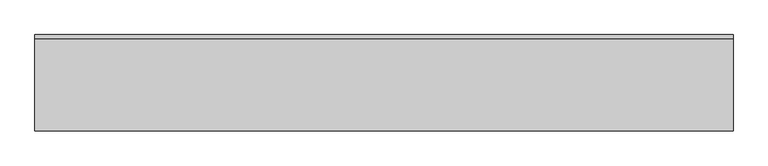
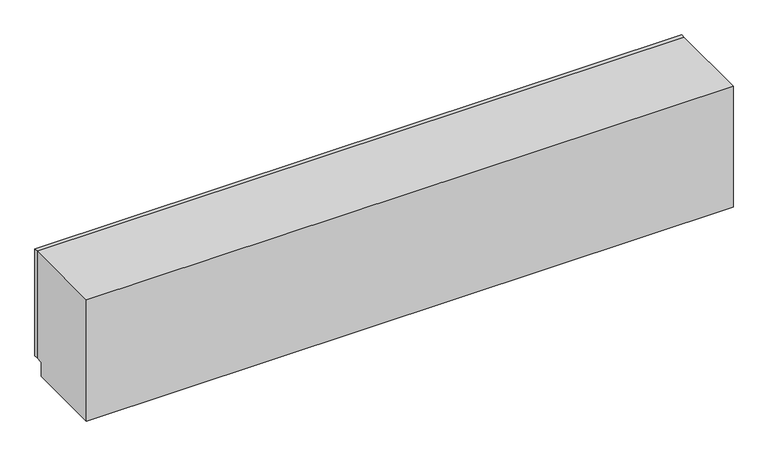
"""IFC4 building model written with IfcOpenShell, lengths in millimetres: furniture geometry, OD_CW_Base Cabinet : OD_CW_Base Cabinet."""

import ifcopenshell
import ifcopenshell.guid

model = None  # the IFC model being written
_history = None  # IfcOwnerHistory: only IFC2X3 demands one
_inside = {}  # id of a spatial element -> (the spatial element, [elements in it])
_under = {}  # id of a project, library or spatial element -> (it, [spatial elements below it])
_declared = {}  # id of a project -> (the project, [libraries it declares])
_typed = {}  # id of a type object -> (the type object, [elements of that type])
_made_of = {}  # id of a material, layer set ... -> (it, [elements and type objects made of it])


def new_model(schema):
    """Start an empty IFC model of exactly this schema.

    Asked for "IFC4X3", IfcOpenShell would pick the latest addendum, in which some entities
    have other attributes; the version numbers below select the first issue.
    IFC2X3 requires an IfcOwnerHistory on every rooted entity: one is made here for all.
    """
    global model, _history
    if schema == "IFC4X3":
        model = ifcopenshell.file(schema_version=(4, 3, 0, 0))
    else:
        model = ifcopenshell.file(schema=schema)
    _inside.clear()
    _under.clear()
    _declared.clear()
    _typed.clear()
    _made_of.clear()
    _history = None
    if model.schema == "IFC2X3":
        org = make("IfcOrganization", Name="unknown")
        user = make(
            "IfcPersonAndOrganization",
            ThePerson=make("IfcPerson", FamilyName="unknown"),
            TheOrganization=org,
        )
        app = make(
            "IfcApplication",
            ApplicationDeveloper=org,
            Version="unknown",
            ApplicationFullName="unknown",
            ApplicationIdentifier="unknown",
        )
        _history = make(
            "IfcOwnerHistory",
            OwningUser=user,
            OwningApplication=app,
            ChangeAction="ADDED",
            CreationDate=0,
        )
    return model


def make(cls, **values):
    """One entity of the class cls with the attributes given. An attribute that is None is left unset."""
    return model.create_entity(
        cls, **{name: value for name, value in values.items() if value is not None}
    )


def rooted(cls, **values):
    """An entity with a GlobalId (a new one), such as an element, a storey or a relation."""
    return make(cls, GlobalId=ifcopenshell.guid.new(), OwnerHistory=_history, **values)


def si_unit(unit_type, name, prefix=None):
    """IfcSIUnit, for example si_unit("LENGTHUNIT", "METRE", prefix="MILLI")."""
    return make("IfcSIUnit", UnitType=unit_type, Prefix=prefix, Name=name)


def assignment(units):
    """IfcUnitAssignment: the units of a project."""
    return None if units is None else make("IfcUnitAssignment", Units=units)


def point(xyz):
    """IfcCartesianPoint."""
    return None if xyz is None else make("IfcCartesianPoint", Coordinates=xyz)


def direction(xyz):
    """IfcDirection."""
    return None if xyz is None else make("IfcDirection", DirectionRatios=xyz)


def frame(location, z_axis=None, x_axis=None):
    """IfcAxis2Placement3D, a coordinate frame: its origin and axes. An axis left out is left unset."""
    return make(
        "IfcAxis2Placement3D",
        Location=point(location),
        Axis=direction(z_axis),
        RefDirection=direction(x_axis),
    )


def origin():
    """The frame at (0, 0, 0) with its axes left unset."""
    return frame((0.0, 0.0, 0.0))


def place(relative_to, where):
    """IfcLocalPlacement: puts the frame where relative to a parent placement (None: the world)."""
    return make(
        "IfcLocalPlacement", PlacementRelTo=relative_to, RelativePlacement=where
    )


def context(
    kind, dimensions, precision=None, world=None, true_north=None, identifier=None
):
    """IfcGeometricRepresentationContext, for example the 3D "Model" context."""
    return make(
        "IfcGeometricRepresentationContext",
        ContextIdentifier=identifier,
        ContextType=kind,
        CoordinateSpaceDimension=dimensions,
        Precision=precision,
        WorldCoordinateSystem=world,
        TrueNorth=true_north,
    )


def project(units=None, contexts=None):
    """IfcProject with its units and contexts."""
    return rooted(
        "IfcProject",
        Name="project",
        RepresentationContexts=contexts,
        UnitsInContext=assignment(units),
    )


def spatial(cls, under=None, at=None, **own):
    """A site, building, storey or space (cls), placed at a placement, below another one or the project."""
    s = rooted(cls, ObjectPlacement=at, **own)
    if under is not None:
        _under.setdefault(under.id(), (under, []))[1].append(s)
    return s


def polyline(points):
    """IfcPolyline through the points."""
    return make("IfcPolyline", Points=[point(p) for p in points])


def outline(outer, holes=None, kind="AREA"):
    """IfcArbitraryClosedProfileDef: a profile drawn as a closed curve; with holes, ...WithVoids."""
    if holes is None:
        return make("IfcArbitraryClosedProfileDef", ProfileType=kind, OuterCurve=outer)
    return make(
        "IfcArbitraryProfileDefWithVoids",
        ProfileType=kind,
        OuterCurve=outer,
        InnerCurves=holes,
    )


def extrude(swept, where, along, depth):
    """IfcExtrudedAreaSolid: the profile swept, set in the frame where, extruded along a direction by depth."""
    return make(
        "IfcExtrudedAreaSolid",
        SweptArea=swept,
        Position=where,
        ExtrudedDirection=direction(along),
        Depth=depth,
    )


def shape(context_of_items, identifier, shape_type, items):
    """IfcShapeRepresentation: the items that make up one representation, for example the "Body"."""
    return make(
        "IfcShapeRepresentation",
        ContextOfItems=context_of_items,
        RepresentationIdentifier=identifier,
        RepresentationType=shape_type,
        Items=items,
    )


def source(mapping_origin, context_of_items, identifier, shape_type, items):
    """IfcRepresentationMap: a shape defined once, which mapped items show again and again."""
    return make(
        "IfcRepresentationMap",
        MappingOrigin=mapping_origin,
        MappedRepresentation=shape(context_of_items, identifier, shape_type, items),
    )


def transform(
    local_origin,
    x_axis=None,
    y_axis=None,
    z_axis=None,
    scale=None,
    scale2=None,
    scale3=None,
    uniform=True,
):
    """IfcCartesianTransformationOperator3D, or its non-uniform kind. x_axis, y_axis, z_axis: its Axis1, 2, 3."""
    if uniform:
        return make(
            "IfcCartesianTransformationOperator3D",
            Axis1=direction(x_axis),
            Axis2=direction(y_axis),
            LocalOrigin=point(local_origin),
            Scale=scale,
            Axis3=direction(z_axis),
        )
    return make(
        "IfcCartesianTransformationOperator3DnonUniform",
        Axis1=direction(x_axis),
        Axis2=direction(y_axis),
        LocalOrigin=point(local_origin),
        Scale=scale,
        Axis3=direction(z_axis),
        Scale2=scale2,
        Scale3=scale3,
    )


def mapped(mapping_source, mapping_target):
    """IfcMappedItem: shows the shape of a source again, moved by a transform."""
    return make(
        "IfcMappedItem", MappingSource=mapping_source, MappingTarget=mapping_target
    )


def made_of(thing, what):
    """Note that an element or type object is made of a material, layer set ...; save() writes the relation."""
    if what is not None:
        _made_of.setdefault(what.id(), (what, []))[1].append(thing)
    return thing


def element(
    cls,
    number,
    at=None,
    inside=None,
    cuts=None,
    type_object=None,
    material=None,
    context=None,
    identifier="Body",
    shape_type=None,
    held_by="IfcProductDefinitionShape",
    body=None,
    shapes=None,
    **own,
):
    """One element of the class cls, such as IfcWall. Its Tag is "e" and its number.

    at: its placement. inside: the storey or other place that contains it. cuts: it is an
    opening in that element (IfcRelVoidsElement). A single representation is given by context,
    identifier, shape_type and body (its items); several are given by shapes. held_by: the class
    of the entity that holds the representations. save() writes the other relations.
    """
    e = rooted(cls, Tag="e%d" % number, ObjectPlacement=at, **own)
    if body is not None:
        shapes = [shape(context, identifier, shape_type, body)]
    if shapes is not None:
        e.Representation = make(held_by, Representations=shapes)
    if inside is not None:
        _inside.setdefault(inside.id(), (inside, []))[1].append(e)
    if cuts is not None:
        rooted(
            "IfcRelVoidsElement", RelatingBuildingElement=cuts, RelatedOpeningElement=e
        )
    if type_object is not None:
        _typed.setdefault(type_object.id(), (type_object, []))[1].append(e)
    return made_of(e, material)


def aggregate(whole, parts):
    """IfcRelAggregates: a whole, such as a stair, and the parts it consists of."""
    return rooted("IfcRelAggregates", RelatingObject=whole, RelatedObjects=parts)


def save(model, path):
    """Write the relations noted so far, then the file.

    IfcRelAggregates (storeys below a building ...), IfcRelContainedInSpatialStructure (elements
    in a storey), IfcRelDefinesByType, IfcRelAssociatesMaterial and IfcRelDeclares: one each for
    every whole, place, type object, material and project.
    """
    for whole, parts in _under.values():
        aggregate(whole, parts)
    for where, things in _inside.values():
        rooted(
            "IfcRelContainedInSpatialStructure",
            RelatedElements=things,
            RelatingStructure=where,
        )
    for kind, things in _typed.values():
        rooted("IfcRelDefinesByType", RelatedObjects=things, RelatingType=kind)
    for what, things in _made_of.values():
        rooted("IfcRelAssociatesMaterial", RelatedObjects=things, RelatingMaterial=what)
    for by, libraries in _declared.values():
        rooted("IfcRelDeclares", RelatingContext=by, RelatedDefinitions=libraries)
    model.write(path)


def furniture_41a9c5b6(model_context):
    return source(origin(), model_context, "Body", "SweptSolid", [
        extrude(outline(polyline([(18.7377049, -25.4), (18.7377049, 0.0), (4438.3377049, 0.0), (4438.3377049, -25.4), (18.7377049, -25.4)])), frame((0.0, 0.0, 101.6), z_axis=(0.0, 0.0, 1.0), x_axis=(1.0, 0.0, 0.0)), (0.0, 0.0, 1.0), 774.7),
        extrude(outline(polyline([(-25.4, 876.3), (-25.4, 101.6), (-76.2, 101.6), (-76.2, 0.0), (-609.6, 0.0), (-609.6, 876.3), (-25.4, 876.3)])), frame((18.7377049, 0.0, 0.0), z_axis=(1.0, 0.0, 0.0), x_axis=(0.0, 1.0, 0.0)), (0.0, 0.0, 1.0), 4419.6),
    ])


if __name__ == "__main__":
    model = new_model("IFC4")
    model_context = context("Model", 3, world=origin())
    ifc_project = project(units=[si_unit("LENGTHUNIT", "METRE", prefix="MILLI")], contexts=[model_context])
    site = spatial("IfcSite", under=ifc_project)
    building = spatial("IfcBuilding", under=site)
    placement = place(None, origin())
    furniture_shape = furniture_41a9c5b6(model_context)
    element("IfcFurniture", 1, ObjectType="OD_CW_Base Cabinet : OD_CW_Base Cabinet", at=placement, inside=building, context=model_context, shape_type="MappedRepresentation", body=[
        mapped(furniture_shape, transform((0.0, 0.0, 0.0), x_axis=(1.0, 0.0, 0.0), y_axis=(0.0, 1.0, 0.0), z_axis=(0.0, 0.0, 1.0))),
    ])
    save(model, "model.ifc")

# Revit data of these elements
# Type "OD_CW_Base Cabinet : OD_CW_Base Cabinet"
#   OD_CW_Width [instance default] = 2' - 10"
#   OD_CW_Length [instance default] = 8' - 0"
#   OD_CW_Height [instance default] = 2' - 3"
#   Depth = 2' - 0"
#   Height = 3' - 0"
#   Width = 4' - 0"
#   OD_CW_Material_Front Panel [instance default] = none
#   OD_CW_Material_Body [instance default] = none
# Element 1 (IfcFurniture, "OD_CW_Base Cabinet : OD_CW_Base Cabinet")
#   OD_CW_Width = 2' - 0"
#   OD_CW_Length = 14' - 6"
#   OD_CW_Height = 2' - 10 1/2"
#   Materials on its faces: "CASEWORK"
# Materials
#   "CASEWORK": class "Generic", colour RGB 181 181 181, transparency 0, Cost = 0
